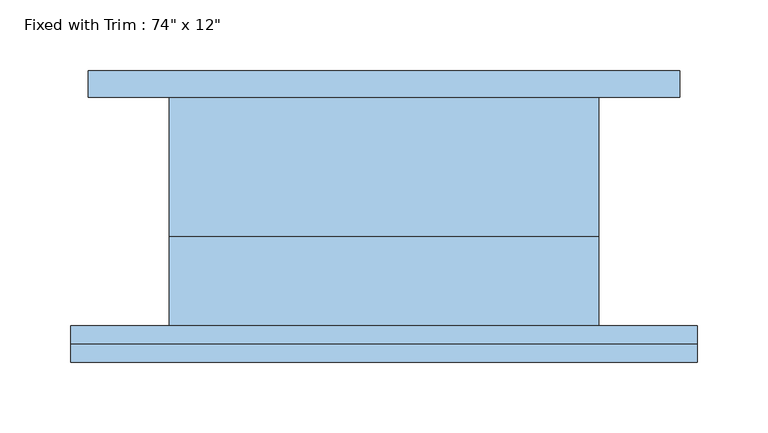
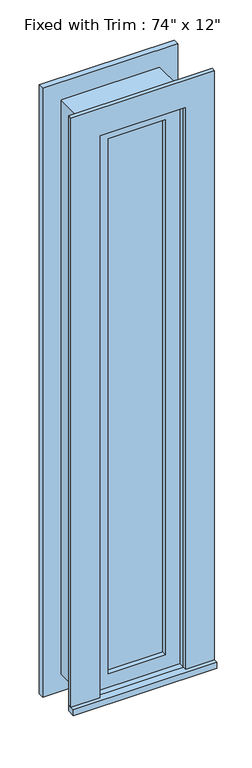
"""IFC4 building model written with IfcOpenShell, lengths in millimetres: window geometry."""

import ifcopenshell
import ifcopenshell.guid

model = None  # the IFC model being written
_history = None  # IfcOwnerHistory: only IFC2X3 demands one
_inside = {}  # id of a spatial element -> (the spatial element, [elements in it])
_under = {}  # id of a project, library or spatial element -> (it, [spatial elements below it])
_declared = {}  # id of a project -> (the project, [libraries it declares])
_typed = {}  # id of a type object -> (the type object, [elements of that type])
_made_of = {}  # id of a material, layer set ... -> (it, [elements and type objects made of it])


def new_model(schema):
    """Start an empty IFC model of exactly this schema.

    Asked for "IFC4X3", IfcOpenShell would pick the latest addendum, in which some entities
    have other attributes; the version numbers below select the first issue.
    IFC2X3 requires an IfcOwnerHistory on every rooted entity: one is made here for all.
    """
    global model, _history
    if schema == "IFC4X3":
        model = ifcopenshell.file(schema_version=(4, 3, 0, 0))
    else:
        model = ifcopenshell.file(schema=schema)
    _inside.clear()
    _under.clear()
    _declared.clear()
    _typed.clear()
    _made_of.clear()
    _history = None
    if model.schema == "IFC2X3":
        org = make("IfcOrganization", Name="unknown")
        user = make(
            "IfcPersonAndOrganization",
            ThePerson=make("IfcPerson", FamilyName="unknown"),
            TheOrganization=org,
        )
        app = make(
            "IfcApplication",
            ApplicationDeveloper=org,
            Version="unknown",
            ApplicationFullName="unknown",
            ApplicationIdentifier="unknown",
        )
        _history = make(
            "IfcOwnerHistory",
            OwningUser=user,
            OwningApplication=app,
            ChangeAction="ADDED",
            CreationDate=0,
        )
    return model


def make(cls, **values):
    """One entity of the class cls with the attributes given. An attribute that is None is left unset."""
    return model.create_entity(
        cls, **{name: value for name, value in values.items() if value is not None}
    )


def rooted(cls, **values):
    """An entity with a GlobalId (a new one), such as an element, a storey or a relation."""
    return make(cls, GlobalId=ifcopenshell.guid.new(), OwnerHistory=_history, **values)


def si_unit(unit_type, name, prefix=None):
    """IfcSIUnit, for example si_unit("LENGTHUNIT", "METRE", prefix="MILLI")."""
    return make("IfcSIUnit", UnitType=unit_type, Prefix=prefix, Name=name)


def assignment(units):
    """IfcUnitAssignment: the units of a project."""
    return None if units is None else make("IfcUnitAssignment", Units=units)


def point(xyz):
    """IfcCartesianPoint."""
    return None if xyz is None else make("IfcCartesianPoint", Coordinates=xyz)


def direction(xyz):
    """IfcDirection."""
    return None if xyz is None else make("IfcDirection", DirectionRatios=xyz)


def frame(location, z_axis=None, x_axis=None):
    """IfcAxis2Placement3D, a coordinate frame: its origin and axes. An axis left out is left unset."""
    return make(
        "IfcAxis2Placement3D",
        Location=point(location),
        Axis=direction(z_axis),
        RefDirection=direction(x_axis),
    )


def origin():
    """The frame at (0, 0, 0) with its axes left unset."""
    return frame((0.0, 0.0, 0.0))


def place(relative_to, where):
    """IfcLocalPlacement: puts the frame where relative to a parent placement (None: the world)."""
    return make(
        "IfcLocalPlacement", PlacementRelTo=relative_to, RelativePlacement=where
    )


def context(
    kind, dimensions, precision=None, world=None, true_north=None, identifier=None
):
    """IfcGeometricRepresentationContext, for example the 3D "Model" context."""
    return make(
        "IfcGeometricRepresentationContext",
        ContextIdentifier=identifier,
        ContextType=kind,
        CoordinateSpaceDimension=dimensions,
        Precision=precision,
        WorldCoordinateSystem=world,
        TrueNorth=true_north,
    )


def project(units=None, contexts=None):
    """IfcProject with its units and contexts."""
    return rooted(
        "IfcProject",
        Name="project",
        RepresentationContexts=contexts,
        UnitsInContext=assignment(units),
    )


def spatial(cls, under=None, at=None, **own):
    """A site, building, storey or space (cls), placed at a placement, below another one or the project."""
    s = rooted(cls, ObjectPlacement=at, **own)
    if under is not None:
        _under.setdefault(under.id(), (under, []))[1].append(s)
    return s


def polyline(points):
    """IfcPolyline through the points."""
    return make("IfcPolyline", Points=[point(p) for p in points])


def outline(outer, holes=None, kind="AREA"):
    """IfcArbitraryClosedProfileDef: a profile drawn as a closed curve; with holes, ...WithVoids."""
    if holes is None:
        return make("IfcArbitraryClosedProfileDef", ProfileType=kind, OuterCurve=outer)
    return make(
        "IfcArbitraryProfileDefWithVoids",
        ProfileType=kind,
        OuterCurve=outer,
        InnerCurves=holes,
    )


def extrude(swept, where, along, depth):
    """IfcExtrudedAreaSolid: the profile swept, set in the frame where, extruded along a direction by depth."""
    return make(
        "IfcExtrudedAreaSolid",
        SweptArea=swept,
        Position=where,
        ExtrudedDirection=direction(along),
        Depth=depth,
    )


def shape(context_of_items, identifier, shape_type, items):
    """IfcShapeRepresentation: the items that make up one representation, for example the "Body"."""
    return make(
        "IfcShapeRepresentation",
        ContextOfItems=context_of_items,
        RepresentationIdentifier=identifier,
        RepresentationType=shape_type,
        Items=items,
    )


def source(mapping_origin, context_of_items, identifier, shape_type, items):
    """IfcRepresentationMap: a shape defined once, which mapped items show again and again."""
    return make(
        "IfcRepresentationMap",
        MappingOrigin=mapping_origin,
        MappedRepresentation=shape(context_of_items, identifier, shape_type, items),
    )


def transform(
    local_origin,
    x_axis=None,
    y_axis=None,
    z_axis=None,
    scale=None,
    scale2=None,
    scale3=None,
    uniform=True,
):
    """IfcCartesianTransformationOperator3D, or its non-uniform kind. x_axis, y_axis, z_axis: its Axis1, 2, 3."""
    if uniform:
        return make(
            "IfcCartesianTransformationOperator3D",
            Axis1=direction(x_axis),
            Axis2=direction(y_axis),
            LocalOrigin=point(local_origin),
            Scale=scale,
            Axis3=direction(z_axis),
        )
    return make(
        "IfcCartesianTransformationOperator3DnonUniform",
        Axis1=direction(x_axis),
        Axis2=direction(y_axis),
        LocalOrigin=point(local_origin),
        Scale=scale,
        Axis3=direction(z_axis),
        Scale2=scale2,
        Scale3=scale3,
    )


def mapped(mapping_source, mapping_target):
    """IfcMappedItem: shows the shape of a source again, moved by a transform."""
    return make(
        "IfcMappedItem", MappingSource=mapping_source, MappingTarget=mapping_target
    )


def made_of(thing, what):
    """Note that an element or type object is made of a material, layer set ...; save() writes the relation."""
    if what is not None:
        _made_of.setdefault(what.id(), (what, []))[1].append(thing)
    return thing


def element(
    cls,
    number,
    at=None,
    inside=None,
    cuts=None,
    type_object=None,
    material=None,
    context=None,
    identifier="Body",
    shape_type=None,
    held_by="IfcProductDefinitionShape",
    body=None,
    shapes=None,
    **own,
):
    """One element of the class cls, such as IfcWall. Its Tag is "e" and its number.

    at: its placement. inside: the storey or other place that contains it. cuts: it is an
    opening in that element (IfcRelVoidsElement). A single representation is given by context,
    identifier, shape_type and body (its items); several are given by shapes. held_by: the class
    of the entity that holds the representations. save() writes the other relations.
    """
    e = rooted(cls, Tag="e%d" % number, ObjectPlacement=at, **own)
    if body is not None:
        shapes = [shape(context, identifier, shape_type, body)]
    if shapes is not None:
        e.Representation = make(held_by, Representations=shapes)
    if inside is not None:
        _inside.setdefault(inside.id(), (inside, []))[1].append(e)
    if cuts is not None:
        rooted(
            "IfcRelVoidsElement", RelatingBuildingElement=cuts, RelatedOpeningElement=e
        )
    if type_object is not None:
        _typed.setdefault(type_object.id(), (type_object, []))[1].append(e)
    return made_of(e, material)


def aggregate(whole, parts):
    """IfcRelAggregates: a whole, such as a stair, and the parts it consists of."""
    return rooted("IfcRelAggregates", RelatingObject=whole, RelatedObjects=parts)


def save(model, path):
    """Write the relations noted so far, then the file.

    IfcRelAggregates (storeys below a building ...), IfcRelContainedInSpatialStructure (elements
    in a storey), IfcRelDefinesByType, IfcRelAssociatesMaterial and IfcRelDeclares: one each for
    every whole, place, type object, material and project.
    """
    for whole, parts in _under.values():
        aggregate(whole, parts)
    for where, things in _inside.values():
        rooted(
            "IfcRelContainedInSpatialStructure",
            RelatedElements=things,
            RelatingStructure=where,
        )
    for kind, things in _typed.values():
        rooted("IfcRelDefinesByType", RelatedObjects=things, RelatingType=kind)
    for what, things in _made_of.values():
        rooted("IfcRelAssociatesMaterial", RelatedObjects=things, RelatingMaterial=what)
    for by, libraries in _declared.values():
        rooted("IfcRelDeclares", RelatingContext=by, RelatedDefinitions=libraries)
    model.write(path)


def window_4a043cc9(model_context):
    return source(origin(), model_context, "Body", "SweptSolid", [
        extrude(outline(polyline([(-260.35, -106.3625), (-260.35, -80.9625), (184.15, -80.9625), (184.15, -106.3625), (-260.35, -106.3625)])), frame((0.0, 0.0, 914.4), z_axis=(0.0, 0.0, 1.0), x_axis=(1.0, 0.0, 0.0)), (0.0, 0.0, 1.0), 19.05),
        extrude(outline(polyline([(2774.95, -171.45), (2774.95, 95.25), (933.45, 95.25), (933.45, 184.15), (2863.85, 184.15), (2863.85, -260.35), (933.45, -260.35), (933.45, -171.45), (2774.95, -171.45)])), frame((0.0, -93.6625, 0.0), z_axis=(0.0, 1.0, 0.0), x_axis=(0.0, 0.0, 1.0)), (0.0, 0.0, 1.0), 12.7),
        extrude(outline(polyline([(2851.15, 171.45), (2851.15, -247.65), (857.25, -247.65), (857.25, 171.45), (2851.15, 171.45)]), holes=[polyline([(2762.25, 82.55), (946.15, 82.55), (946.15, -158.75), (2762.25, -158.75), (2762.25, 82.55)])]), frame((0.0, 80.9625, 0.0), z_axis=(0.0, 1.0, 0.0), x_axis=(0.0, 0.0, 1.0)), (0.0, 0.0, 1.0), 19.05),
        extrude(outline(polyline([(50.8, -33.3375), (50.8, -46.0375), (-127.0, -46.0375), (-127.0, -33.3375), (50.8, -33.3375)])), frame((0.0, 0.0, 977.9), z_axis=(0.0, 0.0, 1.0), x_axis=(1.0, 0.0, 0.0)), (0.0, 0.0, 1.0), 1752.6),
        extrude(outline(polyline([(2774.95, -171.45), (933.45, -171.45), (933.45, 95.25), (2774.95, 95.25), (2774.95, -171.45)]), holes=[polyline([(2730.5, -127.0), (2730.5, 50.8), (977.9, 50.8), (977.9, -127.0), (2730.5, -127.0)])]), frame((0.0, -61.9125, 0.0), z_axis=(0.0, 1.0, 0.0), x_axis=(0.0, 0.0, 1.0)), (0.0, 0.0, 1.0), 44.45),
        extrude(outline(polyline([(2794.0, -190.5), (914.4, -190.5), (914.4, 114.3), (2794.0, 114.3), (2794.0, -190.5)]), holes=[polyline([(2762.25, -158.75), (2762.25, 82.55), (946.15, 82.55), (946.15, -158.75), (2762.25, -158.75)])]), frame((0.0, -17.4625, 0.0), z_axis=(0.0, 1.0, 0.0), x_axis=(0.0, 0.0, 1.0)), (0.0, 0.0, 1.0), 98.425),
        extrude(outline(polyline([(2794.0, 114.3), (2794.0, -190.5), (914.4, -190.5), (914.4, 114.3), (2794.0, 114.3)]), holes=[polyline([(2774.95, 95.25), (933.45, 95.25), (933.45, -171.45), (2774.95, -171.45), (2774.95, 95.25)])]), frame((0.0, -80.9625, 0.0), z_axis=(0.0, 1.0, 0.0), x_axis=(0.0, 0.0, 1.0)), (0.0, 0.0, 1.0), 63.5),
    ])


if __name__ == "__main__":
    model = new_model("IFC4")
    model_context = context("Model", 3, world=origin())
    ifc_project = project(units=[si_unit("LENGTHUNIT", "METRE", prefix="MILLI")], contexts=[model_context])
    site = spatial("IfcSite", under=ifc_project)
    building = spatial("IfcBuilding", under=site)
    placement = place(None, origin())
    window_shape = window_4a043cc9(model_context)
    element("IfcWindow", 1, ObjectType="Fixed with Trim : 74\" x 12\"", at=placement, inside=building, context=model_context, shape_type="MappedRepresentation", body=[
        mapped(window_shape, transform((0.0, 0.0, 0.0), x_axis=(1.0, 0.0, 0.0), y_axis=(0.0, 1.0, 0.0), z_axis=(0.0, 0.0, 1.0))),
    ])
    save(model, "model.ifc")

# Revit data of these elements
# Type "Fixed with Trim : 74\" x 12\""
#   Type Mark = "60"
#   COBie.Type.CreatedBy = "doug.wood@us.ibm.com"
#   COBie.Type.CreatedOn = "2016-04-14T02:07:26"
#   COBie.Type.Name = "Windows_Fixed with Trim_74\" x 12\"_60"
#   COBie.Type.Category = "23-30 20 17 11 : Fixed Windows"
#   COBie.Type.Description = "Fixed with Trim_74\" x 12\""
#   COBie.Type.Manufacturer = ""
#   COBie.Type.ModelNumber = ""
#   Construction Type Id = "GSP4R"
#   Assembly Code = "B2020100"
#   Analytic Construction = "1/8 in Pilkington single glazing"
#   COBie.Type.ReplacementCost = 0
#   Visual Light Transmittance = 0.9
#   Solar Heat Gain Coefficient = 0.78
#   Heat Transfer Coefficient (U) = 3.6886 W/(m²·K)
#   Height = 6' - 2"
#   Default Sill Height = 3' - 0"
#   Trim Projection - Ext. = 0' - 0 1/2"
#   Trim Projection - Int. = 0' - 0 3/4"
#   Trim Width - Exterior = 0' - 3 1/2"
#   Trim Width - Interior = 0' - 3 1/2"
#   Width = 1' - 0"
#   Window Inset = 0' - 0 3/4"
#   COBie.Type = no
#   Glass Pane Material = Glass
#   Sash Material = Sash - White
#   Trim Exterior Material = Trim - White
#   Trim Interior Material = Trim - White
#   Wall Closure = (empty or 0)
# Element 1 (IfcWindow, "Fixed with Trim : 74\" x 12\"")
#   Materials on its faces: "Sash - White", "Trim - White", "Glass"
# Materials
#   "Glass": class "Glass", colour RGB 0 128 192, transparency 0.75, Description = "Soda Lime Glass", Cost = 0
#   "Sash - White": class "Wood", colour RGB 255 255 255, transparency 0, Cost = 0
#   "Trim - White": class "Wood", colour RGB 255 255 255, transparency 0, Cost = 0
